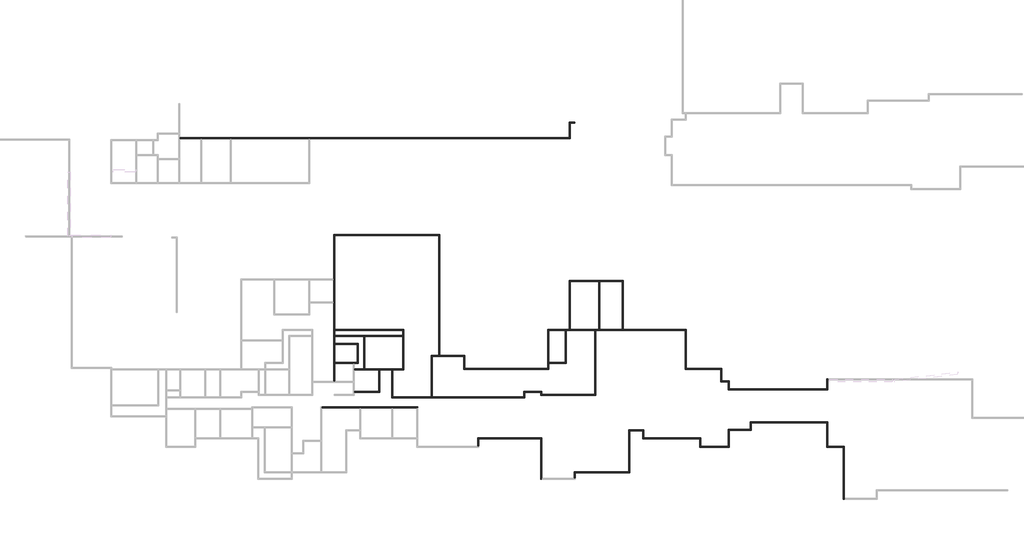
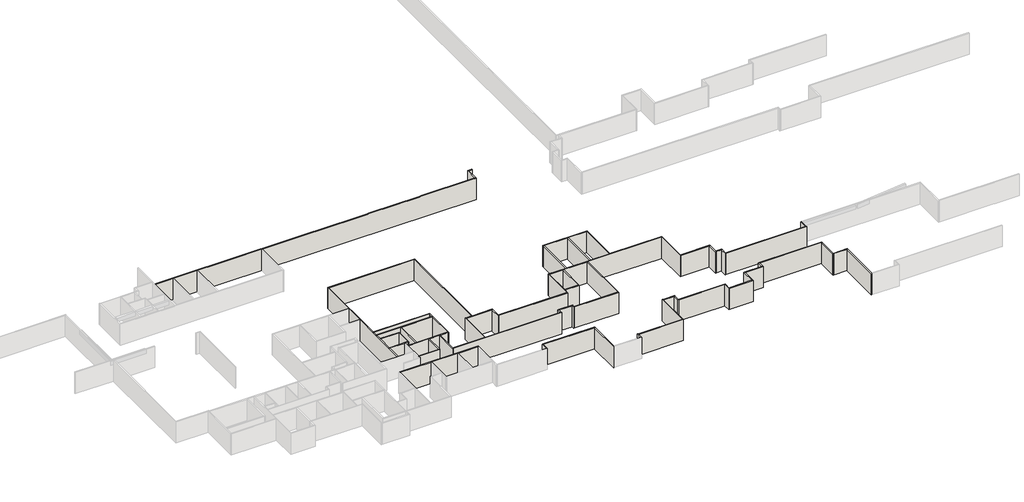
# One storey, part 3 of 8: 61 walls.
"""IFC4 building model written with IfcOpenShell, lengths in millimetres."""

import ifcopenshell
import ifcopenshell.guid

model = None  # the IFC model being written
_history = None  # IfcOwnerHistory: only IFC2X3 demands one
_inside = {}  # id of a spatial element -> (the spatial element, [elements in it])
_under = {}  # id of a project, library or spatial element -> (it, [spatial elements below it])
_declared = {}  # id of a project -> (the project, [libraries it declares])
_typed = {}  # id of a type object -> (the type object, [elements of that type])
_made_of = {}  # id of a material, layer set ... -> (it, [elements and type objects made of it])


def new_model(schema):
    """Start an empty IFC model of exactly this schema.

    Asked for "IFC4X3", IfcOpenShell would pick the latest addendum, in which some entities
    have other attributes; the version numbers below select the first issue.
    IFC2X3 requires an IfcOwnerHistory on every rooted entity: one is made here for all.
    """
    global model, _history
    if schema == "IFC4X3":
        model = ifcopenshell.file(schema_version=(4, 3, 0, 0))
    else:
        model = ifcopenshell.file(schema=schema)
    _inside.clear()
    _under.clear()
    _declared.clear()
    _typed.clear()
    _made_of.clear()
    _history = None
    if model.schema == "IFC2X3":
        org = make("IfcOrganization", Name="unknown")
        user = make(
            "IfcPersonAndOrganization",
            ThePerson=make("IfcPerson", FamilyName="unknown"),
            TheOrganization=org,
        )
        app = make(
            "IfcApplication",
            ApplicationDeveloper=org,
            Version="unknown",
            ApplicationFullName="unknown",
            ApplicationIdentifier="unknown",
        )
        _history = make(
            "IfcOwnerHistory",
            OwningUser=user,
            OwningApplication=app,
            ChangeAction="ADDED",
            CreationDate=0,
        )
    return model


def make(cls, **values):
    """One entity of the class cls with the attributes given. An attribute that is None is left unset."""
    return model.create_entity(
        cls, **{name: value for name, value in values.items() if value is not None}
    )


def rooted(cls, **values):
    """An entity with a GlobalId (a new one), such as an element, a storey or a relation."""
    return make(cls, GlobalId=ifcopenshell.guid.new(), OwnerHistory=_history, **values)


def si_unit(unit_type, name, prefix=None):
    """IfcSIUnit, for example si_unit("LENGTHUNIT", "METRE", prefix="MILLI")."""
    return make("IfcSIUnit", UnitType=unit_type, Prefix=prefix, Name=name)


def assignment(units):
    """IfcUnitAssignment: the units of a project."""
    return None if units is None else make("IfcUnitAssignment", Units=units)


def point(xyz):
    """IfcCartesianPoint."""
    return None if xyz is None else make("IfcCartesianPoint", Coordinates=xyz)


def direction(xyz):
    """IfcDirection."""
    return None if xyz is None else make("IfcDirection", DirectionRatios=xyz)


def frame(location, z_axis=None, x_axis=None):
    """IfcAxis2Placement3D, a coordinate frame: its origin and axes. An axis left out is left unset."""
    return make(
        "IfcAxis2Placement3D",
        Location=point(location),
        Axis=direction(z_axis),
        RefDirection=direction(x_axis),
    )


def origin():
    """The frame at (0, 0, 0) with its axes left unset."""
    return frame((0.0, 0.0, 0.0))


def origin_with_axes():
    """The frame at (0, 0, 0) with the z axis (0, 0, 1) and the x axis (1, 0, 0) written out."""
    return frame((0.0, 0.0, 0.0), z_axis=(0.0, 0.0, 1.0), x_axis=(1.0, 0.0, 0.0))


def place(relative_to, where):
    """IfcLocalPlacement: puts the frame where relative to a parent placement (None: the world)."""
    return make(
        "IfcLocalPlacement", PlacementRelTo=relative_to, RelativePlacement=where
    )


def context(
    kind, dimensions, precision=None, world=None, true_north=None, identifier=None
):
    """IfcGeometricRepresentationContext, for example the 3D "Model" context."""
    return make(
        "IfcGeometricRepresentationContext",
        ContextIdentifier=identifier,
        ContextType=kind,
        CoordinateSpaceDimension=dimensions,
        Precision=precision,
        WorldCoordinateSystem=world,
        TrueNorth=true_north,
    )


def project(units=None, contexts=None):
    """IfcProject with its units and contexts."""
    return rooted(
        "IfcProject",
        Name="project",
        RepresentationContexts=contexts,
        UnitsInContext=assignment(units),
    )


def spatial(cls, under=None, at=None, **own):
    """A site, building, storey or space (cls), placed at a placement, below another one or the project."""
    s = rooted(cls, ObjectPlacement=at, **own)
    if under is not None:
        _under.setdefault(under.id(), (under, []))[1].append(s)
    return s


def polyline(points):
    """IfcPolyline through the points."""
    return make("IfcPolyline", Points=[point(p) for p in points])


def outline(outer, holes=None, kind="AREA"):
    """IfcArbitraryClosedProfileDef: a profile drawn as a closed curve; with holes, ...WithVoids."""
    if holes is None:
        return make("IfcArbitraryClosedProfileDef", ProfileType=kind, OuterCurve=outer)
    return make(
        "IfcArbitraryProfileDefWithVoids",
        ProfileType=kind,
        OuterCurve=outer,
        InnerCurves=holes,
    )


def extrude(swept, where, along, depth):
    """IfcExtrudedAreaSolid: the profile swept, set in the frame where, extruded along a direction by depth."""
    return make(
        "IfcExtrudedAreaSolid",
        SweptArea=swept,
        Position=where,
        ExtrudedDirection=direction(along),
        Depth=depth,
    )


def faces_of(points, faces, orient=None, outer=None):
    """IfcFace entities. A face is a list of loops; a loop is a list of indices into points, from 0.

    orient and outer hold one flag for each loop. By default every Orientation is true, the
    first loop of a face is its IfcFaceOuterBound and the others are IfcFaceBound.
    """
    made = []
    for i, loops in enumerate(faces):
        bounds = []
        for j, loop in enumerate(loops):
            is_outer = j == 0 if outer is None else outer[i][j]
            bounds.append(
                make(
                    "IfcFaceOuterBound" if is_outer else "IfcFaceBound",
                    Bound=make("IfcPolyLoop", Polygon=[points[k] for k in loop]),
                    Orientation=True if orient is None else orient[i][j],
                )
            )
        made.append(make("IfcFace", Bounds=bounds))
    return made


def faceted_brep(points, faces, orient=None, outer=None, voids=None):
    """IfcFacetedBrep: a solid bounded by flat faces; with voids (closed shells), ...WithVoids."""
    shared = [point(p) for p in points]
    hull = make("IfcClosedShell", CfsFaces=faces_of(shared, faces, orient, outer))
    if voids is None:
        return make("IfcFacetedBrep", Outer=hull)
    return make(
        "IfcFacetedBrepWithVoids",
        Outer=hull,
        Voids=[
            make(cls, CfsFaces=faces_of(shared, fs, o, b)) for cls, fs, o, b in voids
        ],
    )


def shape(context_of_items, identifier, shape_type, items):
    """IfcShapeRepresentation: the items that make up one representation, for example the "Body"."""
    return make(
        "IfcShapeRepresentation",
        ContextOfItems=context_of_items,
        RepresentationIdentifier=identifier,
        RepresentationType=shape_type,
        Items=items,
    )


def made_of(thing, what):
    """Note that an element or type object is made of a material, layer set ...; save() writes the relation."""
    if what is not None:
        _made_of.setdefault(what.id(), (what, []))[1].append(thing)
    return thing


def element(
    cls,
    number,
    at=None,
    inside=None,
    cuts=None,
    type_object=None,
    material=None,
    context=None,
    identifier="Body",
    shape_type=None,
    held_by="IfcProductDefinitionShape",
    body=None,
    shapes=None,
    **own,
):
    """One element of the class cls, such as IfcWall. Its Tag is "e" and its number.

    at: its placement. inside: the storey or other place that contains it. cuts: it is an
    opening in that element (IfcRelVoidsElement). A single representation is given by context,
    identifier, shape_type and body (its items); several are given by shapes. held_by: the class
    of the entity that holds the representations. save() writes the other relations.
    """
    e = rooted(cls, Tag="e%d" % number, ObjectPlacement=at, **own)
    if body is not None:
        shapes = [shape(context, identifier, shape_type, body)]
    if shapes is not None:
        e.Representation = make(held_by, Representations=shapes)
    if inside is not None:
        _inside.setdefault(inside.id(), (inside, []))[1].append(e)
    if cuts is not None:
        rooted(
            "IfcRelVoidsElement", RelatingBuildingElement=cuts, RelatedOpeningElement=e
        )
    if type_object is not None:
        _typed.setdefault(type_object.id(), (type_object, []))[1].append(e)
    return made_of(e, material)


def aggregate(whole, parts):
    """IfcRelAggregates: a whole, such as a stair, and the parts it consists of."""
    return rooted("IfcRelAggregates", RelatingObject=whole, RelatedObjects=parts)


def save(model, path):
    """Write the relations noted so far, then the file.

    IfcRelAggregates (storeys below a building ...), IfcRelContainedInSpatialStructure (elements
    in a storey), IfcRelDefinesByType, IfcRelAssociatesMaterial and IfcRelDeclares: one each for
    every whole, place, type object, material and project.
    """
    for whole, parts in _under.values():
        aggregate(whole, parts)
    for where, things in _inside.values():
        rooted(
            "IfcRelContainedInSpatialStructure",
            RelatedElements=things,
            RelatingStructure=where,
        )
    for kind, things in _typed.values():
        rooted("IfcRelDefinesByType", RelatedObjects=things, RelatingType=kind)
    for what, things in _made_of.values():
        rooted("IfcRelAssociatesMaterial", RelatedObjects=things, RelatingMaterial=what)
    for by, libraries in _declared.values():
        rooted("IfcRelDeclares", RelatingContext=by, RelatedDefinitions=libraries)
    model.write(path)


model = new_model("IFC4")

# Units and contexts
model_context = context("Model", 3, world=origin())
ifc_project = project(units=[si_unit("LENGTHUNIT", "METRE", prefix="MILLI")], contexts=[model_context])

# Site, building, storey
site = spatial("IfcSite", under=ifc_project)
building = spatial("IfcBuilding", under=site)
storey = spatial("IfcBuildingStorey", under=building, Name="户型图", Elevation=0.0)

# Walls
placement = place(None, origin())
element("IfcWall", 1, ObjectType="所有墙体", at=placement, inside=storey, context=model_context, shape_type="Brep", body=[
    faceted_brep([(146227.9809999, 19565.6854079, 0.0), (146227.9809999, 20445.6854108, 0.0), (146227.9809999, 20565.6854108, 0.0), (146227.9809999, 20565.6854108, 3300.0), (146227.9809999, 20445.6854108, 3300.0), (146227.9809999, 19565.6854079, 3300.0), (146107.9809999, 19565.6854079, 0.0), (146107.9809999, 19565.6854079, 3300.0), (146107.9809999, 20565.6854108, 3300.0), (146107.9809999, 20565.6854108, 0.0)], [[[0, 1, 2, 3, 4, 5]], [[6, 7, 8, 9]], [[2, 1, 0, 6, 9]], [[5, 4, 3, 8, 7]], [[0, 5, 7, 6]], [[3, 2, 9, 8]]]),
])
element("IfcWall", 2, ObjectType="所有墙体", at=placement, inside=storey, context=model_context, shape_type="Brep", body=[
    faceted_brep([(146227.9809999, 20445.6854108, 0.0), (153757.9809859, 20445.6854108, 0.0), (153877.9809859, 20445.6854108, 0.0), (153877.9809859, 20445.6854108, 3300.0), (153757.9809859, 20445.6854108, 3300.0), (146227.9809999, 20445.6854108, 3300.0), (146227.9809999, 20565.6854108, 0.0), (146227.9809999, 20565.6854108, 3300.0), (153877.9809859, 20565.6854108, 3300.0), (153877.9809859, 20565.6854108, 0.0)], [[[0, 1, 2, 3, 4, 5]], [[6, 7, 8, 9]], [[2, 1, 0, 6, 9]], [[5, 4, 3, 8, 7]], [[0, 5, 7, 6]], [[3, 2, 9, 8]]]),
])
element("IfcWall", 3, ObjectType="所有墙体", at=placement, inside=storey, context=model_context, shape_type="Brep", body=[
    faceted_brep([(153757.9809859, 20445.6854108, 0.0), (153757.9809859, 15545.6854108, 0.0), (153757.9809859, 15545.6854108, 3300.0), (153757.9809859, 20445.6854108, 3300.0), (153877.9809859, 20445.6854108, 0.0), (153877.9809859, 20445.6854108, 3300.0), (153877.9809859, 15665.6854108, 3300.0), (153877.9809859, 15545.6854108, 3300.0), (153877.9809859, 15545.6854108, 0.0), (153877.9809859, 15665.6854108, 0.0)], [[[0, 1, 2, 3]], [[4, 5, 6, 7, 8, 9]], [[1, 0, 4, 9, 8]], [[3, 2, 7, 6, 5]], [[0, 3, 5, 4]], [[2, 1, 8, 7]]]),
])
element("IfcWall", 4, ObjectType="所有墙体", at=placement, inside=storey, context=model_context, shape_type="Brep", body=[
    faceted_brep([(157927.981003, 15665.6854108, 0.0), (157927.981003, 16345.6854097, 0.0), (157927.981003, 16465.6854097, 0.0), (157927.981003, 16465.6854097, 3300.0), (157927.981003, 16345.6854097, 3300.0), (157927.981003, 15665.6854108, 3300.0), (157807.981003, 15665.6854108, 0.0), (157807.981003, 15665.6854108, 3300.0), (157807.981003, 16465.6854097, 3300.0), (157807.981003, 16465.6854097, 0.0)], [[[0, 1, 2, 3, 4, 5]], [[6, 7, 8, 9]], [[2, 1, 0, 6, 9]], [[5, 4, 3, 8, 7]], [[0, 5, 7, 6]], [[3, 2, 9, 8]]]),
])
element("IfcWall", 5, ObjectType="所有墙体", at=placement, inside=storey, context=model_context, shape_type="Brep", body=[
    faceted_brep([(157927.981003, 16345.6854097, 0.0), (164527.9809935, 16345.6854097, 0.0), (164527.9809935, 16345.6854097, 3300.0), (157927.981003, 16345.6854097, 3300.0), (157927.981003, 16465.6854097, 0.0), (157927.981003, 16465.6854097, 3300.0), (164407.9809935, 16465.6854097, 3300.0), (164527.9809935, 16465.6854097, 3300.0), (164527.9809935, 16465.6854097, 0.0), (164407.9809935, 16465.6854097, 0.0)], [[[0, 1, 2, 3]], [[4, 5, 6, 7, 8, 9]], [[1, 0, 4, 9, 8]], [[3, 2, 7, 6, 5]], [[0, 3, 5, 4]], [[2, 1, 8, 7]]]),
])
element("IfcWall", 6, ObjectType="所有墙体", at=placement, inside=storey, context=model_context, shape_type="Brep", body=[
    faceted_brep([(164527.9809935, 16465.6854097, 0.0), (164527.9809935, 21420.9349261, 0.0), (164527.9809935, 21540.9349261, 0.0), (164527.9809935, 21540.9349261, 3300.0), (164527.9809935, 21420.9349261, 3300.0), (164527.9809935, 16465.6854097, 3300.0), (164407.9809935, 16465.6854097, 0.0), (164407.9809935, 16465.6854097, 3300.0), (164407.9809935, 21540.9349261, 3300.0), (164407.9809935, 21540.9349261, 0.0)], [[[0, 1, 2, 3, 4, 5]], [[6, 7, 8, 9]], [[2, 1, 0, 6, 9]], [[5, 4, 3, 8, 7]], [[0, 5, 7, 6]], [[3, 2, 9, 8]]]),
])
element("IfcWall", 7, ObjectType="所有墙体", at=placement, inside=storey, context=model_context, shape_type="Brep", body=[
    faceted_brep([(164527.9809935, 21420.9349261, 0.0), (166107.9809965, 21420.9349261, 0.0), (166227.9809965, 21420.9349261, 0.0), (166227.9809965, 21420.9349261, 3300.0), (166107.9809965, 21420.9349261, 3300.0), (164527.9809935, 21420.9349261, 3300.0), (164527.9809935, 21540.9349261, 0.0), (164527.9809935, 21540.9349261, 3300.0), (166227.9809965, 21540.9349261, 3300.0), (166227.9809965, 21540.9349261, 0.0)], [[[0, 1, 2, 3, 4, 5]], [[6, 7, 8, 9]], [[2, 1, 0, 6, 9]], [[5, 4, 3, 8, 7]], [[0, 5, 7, 6]], [[3, 2, 9, 8]]]),
])
element("IfcWall", 8, ObjectType="所有墙体", at=placement, inside=storey, context=model_context, shape_type="Brep", body=[
    faceted_brep([(166107.9809965, 21420.9349261, 0.0), (166107.9809965, 20445.6854108, 0.0), (166107.9809965, 20445.6854108, 3300.0), (166107.9809965, 21420.9349261, 3300.0), (166227.9809965, 21420.9349261, 0.0), (166227.9809965, 21420.9349261, 3300.0), (166227.9809965, 20565.6854108, 3300.0), (166227.9809965, 20445.6854108, 3300.0), (166227.9809965, 20445.6854108, 0.0), (166227.9809965, 20565.6854108, 0.0)], [[[0, 1, 2, 3]], [[4, 5, 6, 7, 8, 9]], [[1, 0, 4, 9, 8]], [[3, 2, 7, 6, 5]], [[0, 3, 5, 4]], [[2, 1, 8, 7]]]),
])
element("IfcWall", 9, ObjectType="所有墙体", at=placement, inside=storey, context=model_context, shape_type="Brep", body=[
    faceted_brep([(166227.9809965, 20445.6854108, 0.0), (173007.9809872, 20445.6854108, 0.0), (173127.9809872, 20445.6854108, 0.0), (173127.9809872, 20445.6854108, 3300.0), (173007.9809872, 20445.6854108, 3300.0), (166227.9809965, 20445.6854108, 3300.0), (166227.9809965, 20565.6854108, 0.0), (166227.9809965, 20565.6854108, 3300.0), (173127.9809872, 20565.6854108, 3300.0), (173127.9809872, 20565.6854108, 0.0)], [[[0, 1, 2, 3, 4, 5]], [[6, 7, 8, 9]], [[2, 1, 0, 6, 9]], [[5, 4, 3, 8, 7]], [[0, 5, 7, 6]], [[3, 2, 9, 8]]]),
])
element("IfcWall", 10, ObjectType="所有墙体", at=placement, inside=storey, context=model_context, shape_type="Brep", body=[
    faceted_brep([(173007.9809872, 20445.6854108, 0.0), (173007.9809872, 19445.6854134, 0.0), (173007.9809872, 19445.6854134, 3300.0), (173007.9809872, 20445.6854108, 3300.0), (173127.9809872, 20445.6854108, 0.0), (173127.9809872, 20445.6854108, 3300.0), (173127.9809872, 19565.6854134, 3300.0), (173127.9809872, 19445.6854134, 3300.0), (173127.9809872, 19445.6854134, 0.0), (173127.9809872, 19565.6854134, 0.0)], [[[0, 1, 2, 3]], [[4, 5, 6, 7, 8, 9]], [[1, 0, 4, 9, 8]], [[3, 2, 7, 6, 5]], [[0, 3, 5, 4]], [[2, 1, 8, 7]]]),
])
element("IfcWall", 11, ObjectType="所有墙体", at=placement, inside=storey, context=model_context, shape_type="Brep", body=[
    faceted_brep([(173127.9809872, 19445.6854134, 0.0), (176627.9809932, 19445.6854134, 0.0), (176627.9809932, 19445.6854134, 3300.0), (173127.9809872, 19445.6854134, 3300.0), (173127.9809872, 19565.6854134, 0.0), (173127.9809872, 19565.6854134, 3300.0), (176507.9809932, 19565.6854134, 3300.0), (176627.9809932, 19565.6854134, 3300.0), (176627.9809932, 19565.6854134, 0.0), (176507.9809932, 19565.6854134, 0.0)], [[[0, 1, 2, 3]], [[4, 5, 6, 7, 8, 9]], [[1, 0, 4, 9, 8]], [[3, 2, 7, 6, 5]], [[0, 3, 5, 4]], [[2, 1, 8, 7]]]),
])
element("IfcWall", 12, ObjectType="所有墙体", at=placement, inside=storey, context=model_context, shape_type="Brep", body=[
    faceted_brep([(176627.9809932, 19565.6854134, 0.0), (176627.9809932, 21496.1844416, 0.0), (176627.9809932, 21616.1844416, 0.0), (176627.9809932, 21616.1844416, 3300.0), (176627.9809932, 21496.1844416, 3300.0), (176627.9809932, 19565.6854134, 3300.0), (176507.9809932, 19565.6854134, 0.0), (176507.9809932, 19565.6854134, 3300.0), (176507.9809932, 21616.1844416, 3300.0), (176507.9809932, 21616.1844416, 0.0)], [[[0, 1, 2, 3, 4, 5]], [[6, 7, 8, 9]], [[2, 1, 0, 6, 9]], [[5, 4, 3, 8, 7]], [[0, 5, 7, 6]], [[3, 2, 9, 8]]]),
])
element("IfcWall", 13, ObjectType="所有墙体", at=placement, inside=storey, context=model_context, shape_type="Brep", body=[
    faceted_brep([(176627.9809932, 21496.1844416, 0.0), (179277.9850002, 21496.1844416, 0.0), (179277.9850002, 21496.1844416, 3300.0), (176627.9809932, 21496.1844416, 3300.0), (176627.9809932, 21616.1844416, 0.0), (176627.9809932, 21616.1844416, 3300.0), (179157.9850002, 21616.1844416, 3300.0), (179277.9850002, 21616.1844416, 3300.0), (179277.9850002, 21616.1844416, 0.0), (179157.9850002, 21616.1844416, 0.0)], [[[0, 1, 2, 3]], [[4, 5, 6, 7, 8, 9]], [[1, 0, 4, 9, 8]], [[3, 2, 7, 6, 5]], [[0, 3, 5, 4]], [[2, 1, 8, 7]]]),
])
element("IfcWall", 14, ObjectType="所有墙体", at=placement, inside=storey, context=model_context, shape_type="Brep", body=[
    faceted_brep([(179277.9850002, 21616.1844416, 0.0), (179277.9850002, 22396.1673448, 0.0), (179277.9850002, 22516.1673448, 0.0), (179277.9850002, 22516.1673448, 3300.0), (179277.9850002, 22396.1673448, 3300.0), (179277.9850002, 21616.1844416, 3300.0), (179157.9850002, 21616.1844416, 0.0), (179157.9850002, 21616.1844416, 3300.0), (179157.9850002, 22516.1673448, 3300.0), (179157.9850002, 22516.1673448, 0.0)], [[[0, 1, 2, 3, 4, 5]], [[6, 7, 8, 9]], [[2, 1, 0, 6, 9]], [[5, 4, 3, 8, 7]], [[0, 5, 7, 6]], [[3, 2, 9, 8]]]),
])
element("IfcWall", 15, ObjectType="所有墙体", at=placement, inside=storey, context=model_context, shape_type="Brep", body=[
    faceted_brep([(179277.9850002, 22396.1673448, 0.0), (188413.8473665, 22396.1673448, 0.0), (188533.8473665, 22396.1673448, 0.0), (188533.8473665, 22396.1673448, 3300.0), (188413.8473665, 22396.1673448, 3300.0), (179277.9850002, 22396.1673448, 3300.0), (179277.9850002, 22516.1673448, 0.0), (179277.9850002, 22516.1673448, 3300.0), (188533.8473665, 22516.1673448, 3300.0), (188533.8473665, 22516.1673448, 0.0)], [[[0, 1, 2, 3, 4, 5]], [[6, 7, 8, 9]], [[2, 1, 0, 6, 9]], [[5, 4, 3, 8, 7]], [[0, 5, 7, 6]], [[3, 2, 9, 8]]]),
])
element("IfcWall", 16, ObjectType="所有墙体", at=placement, inside=storey, context=model_context, shape_type="Brep", body=[
    faceted_brep([(188413.8473665, 22396.1673448, 0.0), (188413.8473665, 19445.6854134, 0.0), (188413.8473665, 19445.6854134, 3300.0), (188413.8473665, 22396.1673448, 3300.0), (188533.8473665, 22396.1673448, 0.0), (188533.8473665, 22396.1673448, 3300.0), (188533.8473665, 19565.6854134, 3300.0), (188533.8473665, 19445.6854134, 3300.0), (188533.8473665, 19445.6854134, 0.0), (188533.8473665, 19565.6854134, 0.0)], [[[0, 1, 2, 3]], [[4, 5, 6, 7, 8, 9]], [[1, 0, 4, 9, 8]], [[3, 2, 7, 6, 5]], [[0, 3, 5, 4]], [[2, 1, 8, 7]]]),
])
element("IfcWall", 17, ObjectType="所有墙体", at=placement, inside=storey, context=model_context, shape_type="Brep", body=[
    faceted_brep([(188533.8473665, 19445.6854134, 0.0), (190464.1761986, 19445.6854134, 0.0), (190584.1761986, 19445.6854134, 0.0), (190584.1761986, 19445.6854134, 3300.0), (190464.1761986, 19445.6854134, 3300.0), (188533.8473665, 19445.6854134, 3300.0), (188533.8473665, 19565.6854134, 0.0), (188533.8473665, 19565.6854134, 3300.0), (190584.1761986, 19565.6854134, 3300.0), (190584.1761986, 19565.6854134, 0.0)], [[[0, 1, 2, 3, 4, 5]], [[6, 7, 8, 9]], [[2, 1, 0, 6, 9]], [[5, 4, 3, 8, 7]], [[0, 5, 7, 6]], [[3, 2, 9, 8]]]),
])
element("IfcWall", 18, ObjectType="所有墙体", at=placement, inside=storey, context=model_context, shape_type="Brep", body=[
    faceted_brep([(190464.1761986, 19445.6854134, 0.0), (190464.1761986, 13145.7645172, 0.0), (190464.1761986, 13145.7645172, 3300.0), (190464.1761986, 19445.6854134, 3300.0), (190584.1761986, 19445.6854134, 0.0), (190584.1761986, 19445.6854134, 3300.0), (190584.1761986, 13265.7645172, 3300.0), (190584.1761986, 13145.7645172, 3300.0), (190584.1761986, 13145.7645172, 0.0), (190584.1761986, 13265.7645172, 0.0)], [[[0, 1, 2, 3]], [[4, 5, 6, 7, 8, 9]], [[1, 0, 4, 9, 8]], [[3, 2, 7, 6, 5]], [[0, 3, 5, 4]], [[2, 1, 8, 7]]]),
])
element("IfcWall", 19, ObjectType="所有墙体", at=placement, inside=storey, context=model_context, shape_type="Brep", body=[
    faceted_brep([(128682.9654795, 45156.8473862, 0.0), (128802.9654795, 45156.8473862, 0.0), (141413.8359011, 45156.8473862, 0.0), (141533.8359011, 45156.8473862, 0.0), (141533.8359011, 45156.8473862, 3300.0), (141413.8359011, 45156.8473862, 3300.0), (128802.9654795, 45156.8473862, 3300.0), (128682.9654795, 45156.8473862, 3300.0), (128682.9654795, 45276.8473862, 0.0), (128682.9654795, 45276.8473862, 3300.0), (141533.8359011, 45276.8473862, 3300.0), (141533.8359011, 45276.8473862, 0.0)], [[[0, 1, 2, 3, 4, 5, 6, 7]], [[8, 9, 10, 11]], [[3, 2, 1, 0, 8, 11]], [[7, 6, 5, 4, 10, 9]], [[4, 3, 11, 10]], [[0, 7, 9, 8]]]),
])
element("IfcWall", 20, ObjectType="所有墙体", at=placement, inside=storey, context=model_context, shape_type="SweptSolid", body=[
    extrude(outline(polyline([(141413.8359011, 30576.8473862), (141413.8359011, 45156.8473862), (141533.8359011, 45156.8473862), (141533.8359011, 30576.8473862), (141413.8359011, 30576.8473862)])), origin_with_axes(), (0.0, 0.0, 1.0), 3300.0),
])
element("IfcWall", 21, ObjectType="所有墙体", at=placement, inside=storey, context=model_context, shape_type="Brep", body=[
    faceted_brep([(140627.9809914, 30456.8473862, 0.0), (144408.4809802, 30456.8473862, 0.0), (144528.4809802, 30456.8473862, 0.0), (144528.4809802, 30456.8473862, 3300.0), (144408.4809802, 30456.8473862, 3300.0), (140627.9809914, 30456.8473862, 3300.0), (140627.9809914, 30576.8473862, 0.0), (140627.9809914, 30576.8473862, 3300.0), (141413.8359011, 30576.8473862, 3300.0), (141533.8359011, 30576.8473862, 3300.0), (144528.4809802, 30576.8473862, 3300.0), (144528.4809802, 30576.8473862, 0.0), (141533.8359011, 30576.8473862, 0.0), (141413.8359011, 30576.8473862, 0.0)], [[[0, 1, 2, 3, 4, 5]], [[6, 7, 8, 9, 10, 11, 12, 13]], [[2, 1, 0, 6, 13, 12, 11]], [[5, 4, 3, 10, 9, 8, 7]], [[3, 2, 11, 10]], [[0, 5, 7, 6]]]),
])
element("IfcWall", 22, ObjectType="所有墙体", at=placement, inside=storey, context=model_context, shape_type="Brep", body=[
    faceted_brep([(144408.4809802, 30456.8473862, 0.0), (144408.4809802, 28910.6856669, 0.0), (144408.4809802, 28910.6856669, 3300.0), (144408.4809802, 30456.8473862, 3300.0), (144528.4809802, 30456.8473862, 0.0), (144528.4809802, 30456.8473862, 3300.0), (144528.4809802, 29030.6856669, 3300.0), (144528.4809802, 28910.6856669, 3300.0), (144528.4809802, 28910.6856669, 0.0), (144528.4809802, 29030.6856669, 0.0)], [[[0, 1, 2, 3]], [[4, 5, 6, 7, 8, 9]], [[1, 0, 4, 9, 8]], [[3, 2, 7, 6, 5]], [[0, 3, 5, 4]], [[2, 1, 8, 7]]]),
])
element("IfcWall", 23, ObjectType="所有墙体", at=placement, inside=storey, context=model_context, shape_type="Brep", body=[
    faceted_brep([(144528.4809802, 28910.6856669, 0.0), (154728.4809802, 28910.6856669, 0.0), (154728.4809802, 28910.6856669, 3300.0), (144528.4809802, 28910.6856669, 3300.0), (144528.4809802, 29030.6856669, 0.0), (144528.4809802, 29030.6856669, 3300.0), (154608.4809802, 29030.6856669, 3300.0), (154728.4809802, 29030.6856669, 3300.0), (154728.4809802, 29030.6856669, 0.0), (154608.4809802, 29030.6856669, 0.0)], [[[0, 1, 2, 3]], [[4, 5, 6, 7, 8, 9]], [[1, 0, 4, 9, 8]], [[3, 2, 7, 6, 5]], [[0, 3, 5, 4]], [[2, 1, 8, 7]]]),
])
element("IfcWall", 24, ObjectType="所有墙体", at=placement, inside=storey, context=model_context, shape_type="Brep", body=[
    faceted_brep([(154728.4809802, 29030.6856669, 0.0), (154728.4809802, 29595.6854131, 0.0), (154728.4809802, 29715.6854131, 0.0), (154728.4809802, 33645.6854155, 0.0), (154728.4809802, 33645.6854155, 3300.0), (154728.4809802, 29715.6854131, 3300.0), (154728.4809802, 29595.6854131, 3300.0), (154728.4809802, 29030.6856669, 3300.0), (154608.4809802, 29030.6856669, 0.0), (154608.4809802, 29030.6856669, 3300.0), (154608.4809802, 33645.6854155, 3300.0), (154608.4809802, 33645.6854155, 0.0)], [[[0, 1, 2, 3, 4, 5, 6, 7]], [[8, 9, 10, 11]], [[3, 2, 1, 0, 8, 11]], [[7, 6, 5, 4, 10, 9]], [[0, 7, 9, 8]], [[4, 3, 11, 10]]]),
])
element("IfcWall", 25, ObjectType="所有墙体", at=placement, inside=storey, context=model_context, shape_type="Brep", body=[
    faceted_brep([(154728.4809802, 29595.6854131, 0.0), (156827.9809916, 29595.6854131, 0.0), (156827.9809916, 29595.6854131, 3300.0), (154728.4809802, 29595.6854131, 3300.0), (154728.4809802, 29715.6854131, 0.0), (154728.4809802, 29715.6854131, 3300.0), (156707.9809916, 29715.6854131, 3300.0), (156827.9809916, 29715.6854131, 3300.0), (156827.9809916, 29715.6854131, 0.0), (156707.9809916, 29715.6854131, 0.0)], [[[0, 1, 2, 3]], [[4, 5, 6, 7, 8, 9]], [[1, 0, 4, 9, 8]], [[3, 2, 7, 6, 5]], [[0, 3, 5, 4]], [[2, 1, 8, 7]]]),
])
element("IfcWall", 26, ObjectType="所有墙体", at=placement, inside=storey, context=model_context, shape_type="SweptSolid", body=[
    extrude(outline(polyline([(156827.9809916, 33645.6854155), (156827.9809916, 29715.6854131), (156707.9809916, 29715.6854131), (156707.9809916, 33645.6854155), (156827.9809916, 33645.6854155)])), origin_with_axes(), (0.0, 0.0, 1.0), 3300.0),
])
element("IfcWall", 27, ObjectType="所有墙体", at=placement, inside=storey, context=model_context, shape_type="Brep", body=[
    faceted_brep([(171427.9810052, 33765.6854155, 0.0), (163752.9781417, 33765.6854155, 0.0), (163632.9781417, 33765.6854155, 0.0), (160903.0268476, 33765.6854155, 0.0), (160783.0268476, 33765.6854155, 0.0), (157358.8240567, 33765.6854155, 0.0), (157238.8240567, 33765.6854155, 0.0), (154608.4809802, 33765.6854155, 0.0), (154608.4809802, 33765.6854155, 3300.0), (157238.8240567, 33765.6854155, 3300.0), (157358.8240567, 33765.6854155, 3300.0), (160783.0268476, 33765.6854155, 3300.0), (160903.0268476, 33765.6854155, 3300.0), (163632.9781417, 33765.6854155, 3300.0), (163752.9781417, 33765.6854155, 3300.0), (171427.9810052, 33765.6854155, 3300.0), (171427.9810052, 33645.6854155, 0.0), (171427.9810052, 33645.6854155, 3300.0), (171307.9810052, 33645.6854155, 3300.0), (160427.9809891, 33645.6854155, 3300.0), (160307.9809891, 33645.6854155, 3300.0), (156827.9809916, 33645.6854155, 3300.0), (156707.9809916, 33645.6854155, 3300.0), (154728.4809802, 33645.6854155, 3300.0), (154608.4809802, 33645.6854155, 3300.0), (154608.4809802, 33645.6854155, 0.0), (154728.4809802, 33645.6854155, 0.0), (156707.9809916, 33645.6854155, 0.0), (156827.9809916, 33645.6854155, 0.0), (160307.9809891, 33645.6854155, 0.0), (160427.9809891, 33645.6854155, 0.0), (171307.9810052, 33645.6854155, 0.0)], [[[0, 1, 2, 3, 4, 5, 6, 7, 8, 9, 10, 11, 12, 13, 14, 15]], [[16, 17, 18, 19, 20, 21, 22, 23, 24, 25, 26, 27, 28, 29, 30, 31]], [[7, 6, 5, 4, 3, 2, 1, 0, 16, 31, 30, 29, 28, 27, 26, 25]], [[15, 14, 13, 12, 11, 10, 9, 8, 24, 23, 22, 21, 20, 19, 18, 17]], [[8, 7, 25, 24]], [[0, 15, 17, 16]]]),
])
element("IfcWall", 28, ObjectType="所有墙体", at=placement, inside=storey, context=model_context, shape_type="SweptSolid", body=[
    extrude(outline(polyline([(160903.0268476, 39545.6854155), (160903.0268476, 33765.6854155), (160783.0268476, 33765.6854155), (160783.0268476, 39545.6854155), (160903.0268476, 39545.6854155)])), origin_with_axes(), (0.0, 0.0, 1.0), 3300.0),
])
element("IfcWall", 29, ObjectType="所有墙体", at=placement, inside=storey, context=model_context, shape_type="Brep", body=[
    faceted_brep([(163752.9781417, 39665.6854155, 0.0), (157238.8240567, 39665.6854155, 0.0), (157238.8240567, 39665.6854155, 3300.0), (163752.9781417, 39665.6854155, 3300.0), (163752.9781417, 39545.6854155, 0.0), (163752.9781417, 39545.6854155, 3300.0), (163632.9781417, 39545.6854155, 3300.0), (160903.0268476, 39545.6854155, 3300.0), (160783.0268476, 39545.6854155, 3300.0), (157358.8240567, 39545.6854155, 3300.0), (157238.8240567, 39545.6854155, 3300.0), (157238.8240567, 39545.6854155, 0.0), (157358.8240567, 39545.6854155, 0.0), (160783.0268476, 39545.6854155, 0.0), (160903.0268476, 39545.6854155, 0.0), (163632.9781417, 39545.6854155, 0.0)], [[[0, 1, 2, 3]], [[4, 5, 6, 7, 8, 9, 10, 11, 12, 13, 14, 15]], [[1, 0, 4, 15, 14, 13, 12, 11]], [[3, 2, 10, 9, 8, 7, 6, 5]], [[2, 1, 11, 10]], [[0, 3, 5, 4]]]),
])
element("IfcWall", 30, ObjectType="所有墙体", at=placement, inside=storey, context=model_context, shape_type="SweptSolid", body=[
    extrude(outline(polyline([(157238.8240567, 33765.6854155), (157238.8240567, 39545.6854155), (157358.8240567, 39545.6854155), (157358.8240567, 33765.6854155), (157238.8240567, 33765.6854155)])), origin_with_axes(), (0.0, 0.0, 1.0), 3300.0),
])
element("IfcWall", 31, ObjectType="所有墙体", at=placement, inside=storey, context=model_context, shape_type="SweptSolid", body=[
    extrude(outline(polyline([(163632.9781417, 33765.6854155), (163632.9781417, 39545.6854155), (163752.9781417, 39545.6854155), (163752.9781417, 33765.6854155), (163632.9781417, 33765.6854155)])), origin_with_axes(), (0.0, 0.0, 1.0), 3300.0),
])
element("IfcWall", 32, ObjectType="所有墙体", at=placement, inside=storey, context=model_context, shape_type="Brep", body=[
    faceted_brep([(171307.9810052, 33645.6854155, 0.0), (171307.9810052, 28910.6856669, 0.0), (171307.9810052, 28910.6856669, 3300.0), (171307.9810052, 33645.6854155, 3300.0), (171427.9810052, 33645.6854155, 0.0), (171427.9810052, 33645.6854155, 3300.0), (171427.9810052, 29030.6856669, 3300.0), (171427.9810052, 28910.6856669, 3300.0), (171427.9810052, 28910.6856669, 0.0), (171427.9810052, 29030.6856669, 0.0)], [[[0, 1, 2, 3]], [[4, 5, 6, 7, 8, 9]], [[1, 0, 4, 9, 8]], [[3, 2, 7, 6, 5]], [[0, 3, 5, 4]], [[2, 1, 8, 7]]]),
])
element("IfcWall", 33, ObjectType="所有墙体", at=placement, inside=storey, context=model_context, shape_type="Brep", body=[
    faceted_brep([(171427.9810052, 28910.6856669, 0.0), (175607.9810895, 28910.6856669, 0.0), (175727.9810895, 28910.6856669, 0.0), (175727.9810895, 28910.6856669, 3300.0), (175607.9810895, 28910.6856669, 3300.0), (171427.9810052, 28910.6856669, 3300.0), (171427.9810052, 29030.6856669, 0.0), (171427.9810052, 29030.6856669, 3300.0), (175727.9810895, 29030.6856669, 3300.0), (175727.9810895, 29030.6856669, 0.0)], [[[0, 1, 2, 3, 4, 5]], [[6, 7, 8, 9]], [[2, 1, 0, 6, 9]], [[5, 4, 3, 8, 7]], [[0, 5, 7, 6]], [[3, 2, 9, 8]]]),
])
element("IfcWall", 34, ObjectType="所有墙体", at=placement, inside=storey, context=model_context, shape_type="Brep", body=[
    faceted_brep([(175607.9810895, 28910.6856669, 0.0), (175607.9810895, 27370.687934, 0.0), (175607.9810895, 27370.687934, 3300.0), (175607.9810895, 28910.6856669, 3300.0), (175727.9810895, 28910.6856669, 0.0), (175727.9810895, 28910.6856669, 3300.0), (175727.9810895, 27490.687934, 3300.0), (175727.9810895, 27370.687934, 3300.0), (175727.9810895, 27370.687934, 0.0), (175727.9810895, 27490.687934, 0.0)], [[[0, 1, 2, 3]], [[4, 5, 6, 7, 8, 9]], [[1, 0, 4, 9, 8]], [[3, 2, 7, 6, 5]], [[0, 3, 5, 4]], [[2, 1, 8, 7]]]),
])
element("IfcWall", 35, ObjectType="所有墙体", at=placement, inside=storey, context=model_context, shape_type="Brep", body=[
    faceted_brep([(175727.9810895, 27370.687934, 0.0), (176507.9809932, 27370.687934, 0.0), (176627.9809932, 27370.687934, 0.0), (176627.9809932, 27370.687934, 3300.0), (176507.9809932, 27370.687934, 3300.0), (175727.9810895, 27370.687934, 3300.0), (175727.9810895, 27490.687934, 0.0), (175727.9810895, 27490.687934, 3300.0), (176627.9809932, 27490.687934, 3300.0), (176627.9809932, 27490.687934, 0.0)], [[[0, 1, 2, 3, 4, 5]], [[6, 7, 8, 9]], [[2, 1, 0, 6, 9]], [[5, 4, 3, 8, 7]], [[0, 5, 7, 6]], [[3, 2, 9, 8]]]),
])
element("IfcWall", 36, ObjectType="所有墙体", at=placement, inside=storey, context=model_context, shape_type="Brep", body=[
    faceted_brep([(176507.9809932, 27370.687934, 0.0), (176507.9809932, 26395.6879034, 0.0), (176507.9809932, 26395.6879034, 3300.0), (176507.9809932, 27370.687934, 3300.0), (176627.9809932, 27370.687934, 0.0), (176627.9809932, 27370.687934, 3300.0), (176627.9809932, 26515.6879034, 3300.0), (176627.9809932, 26395.6879034, 3300.0), (176627.9809932, 26395.6879034, 0.0), (176627.9809932, 26515.6879034, 0.0)], [[[0, 1, 2, 3]], [[4, 5, 6, 7, 8, 9]], [[1, 0, 4, 9, 8]], [[3, 2, 7, 6, 5]], [[0, 3, 5, 4]], [[2, 1, 8, 7]]]),
])
element("IfcWall", 37, ObjectType="所有墙体", at=placement, inside=storey, context=model_context, shape_type="Brep", body=[
    faceted_brep([(176627.9809932, 26395.6879034, 0.0), (188533.8473665, 26395.6879034, 0.0), (188533.8473665, 26395.6879034, 3300.0), (176627.9809932, 26395.6879034, 3300.0), (176627.9809932, 26515.6879034, 0.0), (176627.9809932, 26515.6879034, 3300.0), (188413.8473665, 26515.6879034, 3300.0), (188533.8473665, 26515.6879034, 3300.0), (188533.8473665, 26515.6879034, 0.0), (188413.8473665, 26515.6879034, 0.0)], [[[0, 1, 2, 3]], [[4, 5, 6, 7, 8, 9]], [[1, 0, 4, 9, 8]], [[3, 2, 7, 6, 5]], [[0, 3, 5, 4]], [[2, 1, 8, 7]]]),
])
element("IfcWall", 38, ObjectType="所有墙体", at=placement, inside=storey, context=model_context, shape_type="Brep", body=[
    faceted_brep([(188533.8473665, 26515.6879034, 0.0), (188533.8473665, 27606.8378863, 0.0), (188533.8473665, 27726.8378863, 0.0), (188533.8473665, 27726.8378863, 3300.0), (188533.8473665, 27606.8378863, 3300.0), (188533.8473665, 26515.6879034, 3300.0), (188413.8473665, 26515.6879034, 0.0), (188413.8473665, 26515.6879034, 3300.0), (188413.8473665, 27726.8378863, 3300.0), (188413.8473665, 27726.8378863, 0.0)], [[[0, 1, 2, 3, 4, 5]], [[6, 7, 8, 9]], [[2, 1, 0, 6, 9]], [[5, 4, 3, 8, 7]], [[0, 5, 7, 6]], [[3, 2, 9, 8]]]),
])
element("IfcWall", 39, ObjectType="所有墙体", at=placement, inside=storey, context=model_context, shape_type="Brep", body=[
    faceted_brep([(128682.9654795, 45156.8473862, 0.0), (128682.9654795, 39876.8473862, 0.0), (128682.9654795, 39756.8473862, 0.0), (128682.9654795, 37051.6496402, 0.0), (128682.9654795, 36931.6496402, 0.0), (128682.9654795, 27451.6496402, 0.0), (128682.9654795, 27451.6496402, 3300.0), (128682.9654795, 36931.6496402, 3300.0), (128682.9654795, 37051.6496402, 3300.0), (128682.9654795, 39756.8473862, 3300.0), (128682.9654795, 39876.8473862, 3300.0), (128682.9654795, 45156.8473862, 3300.0), (128802.9654795, 45156.8473862, 0.0), (128802.9654795, 45156.8473862, 3300.0), (128802.9654795, 33765.6854157, 3300.0), (128802.9654795, 33645.6854157, 3300.0), (128802.9654795, 32990.685413, 3300.0), (128802.9654795, 32870.685413, 3300.0), (128802.9654795, 32040.6854089, 3300.0), (128802.9654795, 31920.6854089, 3300.0), (128802.9654795, 29715.6854131, 3300.0), (128802.9654795, 29595.6854131, 3300.0), (128802.9654795, 27451.6496402, 3300.0), (128802.9654795, 27451.6496402, 0.0), (128802.9654795, 29595.6854131, 0.0), (128802.9654795, 29715.6854131, 0.0), (128802.9654795, 31920.6854089, 0.0), (128802.9654795, 32040.6854089, 0.0), (128802.9654795, 32870.685413, 0.0), (128802.9654795, 32990.685413, 0.0), (128802.9654795, 33645.6854157, 0.0), (128802.9654795, 33765.6854157, 0.0)], [[[0, 1, 2, 3, 4, 5, 6, 7, 8, 9, 10, 11]], [[12, 13, 14, 15, 16, 17, 18, 19, 20, 21, 22, 23, 24, 25, 26, 27, 28, 29, 30, 31]], [[5, 4, 3, 2, 1, 0, 12, 31, 30, 29, 28, 27, 26, 25, 24, 23]], [[11, 10, 9, 8, 7, 6, 22, 21, 20, 19, 18, 17, 16, 15, 14, 13]], [[0, 11, 13, 12]], [[6, 5, 23, 22]]]),
])
element("IfcWall", 40, ObjectType="所有墙体", at=placement, inside=storey, context=model_context, shape_type="Brep", body=[
    faceted_brep([(109958.7128377, 56907.0370398, 0.0), (125638.8240412, 56907.0370398, 0.0), (125758.8240412, 56907.0370398, 0.0), (157358.8240567, 56907.0370398, 0.0), (157358.8240567, 56907.0370398, 3300.0), (157226.4248507, 56907.0370398, 3300.0), (156926.4248507, 56907.0370398, 3300.0), (149326.4248507, 56907.0370398, 3300.0), (149026.4248507, 56907.0370398, 3300.0), (141526.4248507, 56907.0370398, 3300.0), (141226.4248507, 56907.0370398, 3300.0), (133626.4248507, 56907.0370398, 3300.0), (133326.4248507, 56907.0370398, 3300.0), (125848.8240412, 56907.0370398, 3300.0), (125758.8240412, 56907.0370398, 3300.0), (125638.8240412, 56907.0370398, 3300.0), (125548.8240412, 56907.0370398, 3300.0), (117798.8477351, 56907.0370398, 3300.0), (117498.8477351, 56907.0370398, 3300.0), (109958.7128377, 56907.0370398, 3300.0), (109958.7128377, 57027.0370398, 0.0), (109958.7128377, 57027.0370398, 3300.0), (117498.8477351, 57027.0370398, 3300.0), (117798.8477351, 57027.0370398, 3300.0), (125548.8240412, 57027.0370398, 3300.0), (125848.8240412, 57027.0370398, 3300.0), (133326.4248507, 57027.0370398, 3300.0), (133626.4248507, 57027.0370398, 3300.0), (141226.4248507, 57027.0370398, 3300.0), (141526.4248507, 57027.0370398, 3300.0), (149026.4248507, 57027.0370398, 3300.0), (149326.4248507, 57027.0370398, 3300.0), (156926.4248507, 57027.0370398, 3300.0), (157226.4248507, 57027.0370398, 3300.0), (157238.8240567, 57027.0370398, 3300.0), (157358.8240567, 57027.0370398, 3300.0), (157358.8240567, 57027.0370398, 0.0), (157238.8240567, 57027.0370398, 0.0)], [[[0, 1, 2, 3, 4, 5, 6, 7, 8, 9, 10, 11, 12, 13, 14, 15, 16, 17, 18, 19]], [[20, 21, 22, 23, 24, 25, 26, 27, 28, 29, 30, 31, 32, 33, 34, 35, 36, 37]], [[3, 2, 1, 0, 20, 37, 36]], [[19, 18, 17, 16, 15, 14, 13, 12, 11, 10, 9, 8, 7, 6, 5, 4, 35, 34, 33, 32, 31, 30, 29, 28, 27, 26, 25, 24, 23, 22, 21]], [[0, 19, 21, 20]], [[4, 3, 36, 35]]]),
])
element("IfcWall", 41, ObjectType="所有墙体", at=placement, inside=storey, context=model_context, shape_type="Brep", body=[
    faceted_brep([(157358.8240567, 57027.0370398, 0.0), (157358.8240567, 58806.6495108, 0.0), (157358.8240567, 58926.6495108, 0.0), (157358.8240567, 58926.6495108, 3300.0), (157358.8240567, 58806.6495108, 3300.0), (157358.8240567, 57027.0370398, 3300.0), (157238.8240567, 57027.0370398, 0.0), (157238.8240567, 57027.0370398, 3300.0), (157238.8240567, 58926.6495108, 3300.0), (157238.8240567, 58926.6495108, 0.0)], [[[0, 1, 2, 3, 4, 5]], [[6, 7, 8, 9]], [[2, 1, 0, 6, 9]], [[5, 4, 3, 8, 7]], [[0, 5, 7, 6]], [[3, 2, 9, 8]]]),
])
element("IfcWall", 42, ObjectType="所有墙体", at=placement, inside=storey, context=model_context, shape_type="SweptSolid", body=[
    extrude(outline(polyline([(157873.8477306, 58806.6495108), (157358.8240567, 58806.6495108), (157358.8240567, 58926.6495108), (157873.8477306, 58926.6495108), (157873.8477306, 58806.6495108)])), origin_with_axes(), (0.0, 0.0, 1.0), 3300.0),
])
element("IfcWall", 43, ObjectType="所有墙体", at=placement, inside=storey, context=model_context, shape_type="Brep", body=[
    faceted_brep([(131532.9809813, 29715.6854131, 0.0), (128802.9654795, 29715.6854131, 0.0), (128802.9654795, 29715.6854131, 3300.0), (131532.9809813, 29715.6854131, 3300.0), (131532.9809813, 29595.6854131, 0.0), (131532.9809813, 29595.6854131, 3300.0), (131127.9809837, 29595.6854131, 3300.0), (131007.9809837, 29595.6854131, 3300.0), (128802.9654795, 29595.6854131, 3300.0), (128802.9654795, 29595.6854131, 0.0), (131007.9809837, 29595.6854131, 0.0), (131127.9809837, 29595.6854131, 0.0)], [[[0, 1, 2, 3]], [[4, 5, 6, 7, 8, 9, 10, 11]], [[1, 0, 4, 11, 10, 9]], [[3, 2, 8, 7, 6, 5]], [[2, 1, 9, 8]], [[0, 3, 5, 4]]]),
])
element("IfcWall", 44, ObjectType="所有墙体", at=placement, inside=storey, context=model_context, shape_type="Brep", body=[
    faceted_brep([(128802.9654795, 31920.6854089, 0.0), (131532.9809813, 31920.6854089, 0.0), (131652.9809813, 31920.6854089, 0.0), (131652.9809813, 31920.6854089, 3300.0), (131532.9809813, 31920.6854089, 3300.0), (128802.9654795, 31920.6854089, 3300.0), (128802.9654795, 32040.6854089, 0.0), (128802.9654795, 32040.6854089, 3300.0), (131652.9809813, 32040.6854089, 3300.0), (131652.9809813, 32040.6854089, 0.0)], [[[0, 1, 2, 3, 4, 5]], [[6, 7, 8, 9]], [[2, 1, 0, 6, 9]], [[5, 4, 3, 8, 7]], [[0, 5, 7, 6]], [[3, 2, 9, 8]]]),
])
element("IfcWall", 45, ObjectType="所有墙体", at=placement, inside=storey, context=model_context, shape_type="Brep", body=[
    faceted_brep([(131532.9809813, 31920.6854089, 0.0), (131532.9809813, 29715.6854131, 0.0), (131532.9809813, 29595.6854131, 0.0), (131532.9809813, 29595.6854131, 3300.0), (131532.9809813, 29715.6854131, 3300.0), (131532.9809813, 31920.6854089, 3300.0), (131652.9809813, 31920.6854089, 0.0), (131652.9809813, 31920.6854089, 3300.0), (131652.9809813, 29595.6854131, 3300.0), (131652.9809813, 29595.6854131, 0.0)], [[[0, 1, 2, 3, 4, 5]], [[6, 7, 8, 9]], [[2, 1, 0, 6, 9]], [[5, 4, 3, 8, 7]], [[0, 5, 7, 6]], [[3, 2, 9, 8]]]),
])
element("IfcWall", 46, ObjectType="所有墙体", at=placement, inside=storey, context=model_context, shape_type="Brep", body=[
    faceted_brep([(128802.9654795, 33645.6854157, 0.0), (137007.9809818, 33645.6854157, 0.0), (137127.9809818, 33645.6854157, 0.0), (137127.9809818, 33645.6854157, 3300.0), (137007.9809818, 33645.6854157, 3300.0), (128802.9654795, 33645.6854157, 3300.0), (128802.9654795, 33765.6854157, 0.0), (128802.9654795, 33765.6854157, 3300.0), (137127.9809818, 33765.6854157, 3300.0), (137127.9809818, 33765.6854157, 0.0)], [[[0, 1, 2, 3, 4, 5]], [[6, 7, 8, 9]], [[2, 1, 0, 6, 9]], [[5, 4, 3, 8, 7]], [[0, 5, 7, 6]], [[3, 2, 9, 8]]]),
])
element("IfcWall", 47, ObjectType="所有墙体", at=placement, inside=storey, context=model_context, shape_type="Brep", body=[
    faceted_brep([(137007.9809818, 33645.6854157, 0.0), (137007.9809818, 32990.685413, 0.0), (137007.9809818, 32870.685413, 0.0), (137007.9809818, 28976.8473862, 0.0), (137007.9809818, 28856.8473862, 0.0), (137007.9809818, 28856.8473862, 3300.0), (137007.9809818, 28976.8473862, 3300.0), (137007.9809818, 32870.685413, 3300.0), (137007.9809818, 32990.685413, 3300.0), (137007.9809818, 33645.6854157, 3300.0), (137127.9809818, 33645.6854157, 0.0), (137127.9809818, 33645.6854157, 3300.0), (137127.9809818, 28856.8473862, 3300.0), (137127.9809818, 28856.8473862, 0.0)], [[[0, 1, 2, 3, 4, 5, 6, 7, 8, 9]], [[10, 11, 12, 13]], [[4, 3, 2, 1, 0, 10, 13]], [[9, 8, 7, 6, 5, 12, 11]], [[0, 9, 11, 10]], [[5, 4, 13, 12]]]),
])
element("IfcWall", 48, ObjectType="所有墙体", at=placement, inside=storey, context=model_context, shape_type="Brep", body=[
    faceted_brep([(137007.9809818, 28976.8473862, 0.0), (132427.9809928, 28976.8473862, 0.0), (132307.9809928, 28976.8473862, 0.0), (131127.9809837, 28976.8473862, 0.0), (131127.9809837, 28976.8473862, 3300.0), (132307.9809928, 28976.8473862, 3300.0), (132427.9809928, 28976.8473862, 3300.0), (137007.9809818, 28976.8473862, 3300.0), (137007.9809818, 28856.8473862, 0.0), (137007.9809818, 28856.8473862, 3300.0), (135827.98099, 28856.8473862, 3300.0), (135707.98099, 28856.8473862, 3300.0), (134227.9809868, 28856.8473862, 3300.0), (134107.9809868, 28856.8473862, 3300.0), (131127.9809837, 28856.8473862, 3300.0), (131127.9809837, 28856.8473862, 0.0), (134107.9809868, 28856.8473862, 0.0), (134227.9809868, 28856.8473862, 0.0), (135707.98099, 28856.8473862, 0.0), (135827.98099, 28856.8473862, 0.0)], [[[0, 1, 2, 3, 4, 5, 6, 7]], [[8, 9, 10, 11, 12, 13, 14, 15, 16, 17, 18, 19]], [[3, 2, 1, 0, 8, 19, 18, 17, 16, 15]], [[7, 6, 5, 4, 14, 13, 12, 11, 10, 9]], [[0, 7, 9, 8]], [[4, 3, 15, 14]]]),
])
element("IfcWall", 49, ObjectType="所有墙体", at=placement, inside=storey, context=model_context, shape_type="Brep", body=[
    faceted_brep([(128802.9654795, 32870.685413, 0.0), (132307.9809928, 32870.685413, 0.0), (132427.9809928, 32870.685413, 0.0), (137007.9809818, 32870.685413, 0.0), (137007.9809818, 32870.685413, 3300.0), (132427.9809928, 32870.685413, 3300.0), (132307.9809928, 32870.685413, 3300.0), (128802.9654795, 32870.685413, 3300.0), (128802.9654795, 32990.685413, 0.0), (128802.9654795, 32990.685413, 3300.0), (137007.9809818, 32990.685413, 3300.0), (137007.9809818, 32990.685413, 0.0)], [[[0, 1, 2, 3, 4, 5, 6, 7]], [[8, 9, 10, 11]], [[3, 2, 1, 0, 8, 11]], [[7, 6, 5, 4, 10, 9]], [[0, 7, 9, 8]], [[4, 3, 11, 10]]]),
])
element("IfcWall", 50, ObjectType="所有墙体", at=placement, inside=storey, context=model_context, shape_type="SweptSolid", body=[
    extrude(outline(polyline([(132307.9809928, 28976.8473862), (132307.9809928, 32870.685413), (132427.9809928, 32870.685413), (132427.9809928, 28976.8473862), (132307.9809928, 28976.8473862)])), origin_with_axes(), (0.0, 0.0, 1.0), 3300.0),
])
element("IfcWall", 51, ObjectType="所有墙体", at=placement, inside=storey, context=model_context, shape_type="Brep", body=[
    faceted_brep([(131127.9809837, 26125.3729134, 0.0), (134227.9809868, 26125.3729134, 0.0), (134227.9809868, 26125.3729134, 3300.0), (131127.9809837, 26125.3729134, 3300.0), (131127.9809837, 26245.3729134, 0.0), (131127.9809837, 26245.3729134, 3300.0), (134107.9809868, 26245.3729134, 3300.0), (134227.9809868, 26245.3729134, 3300.0), (134227.9809868, 26245.3729134, 0.0), (134107.9809868, 26245.3729134, 0.0)], [[[0, 1, 2, 3]], [[4, 5, 6, 7, 8, 9]], [[1, 0, 4, 9, 8]], [[3, 2, 7, 6, 5]], [[0, 3, 5, 4]], [[2, 1, 8, 7]]]),
])
element("IfcWall", 52, ObjectType="所有墙体", at=placement, inside=storey, context=model_context, shape_type="SweptSolid", body=[
    extrude(outline(polyline([(134227.9809868, 28856.8473862), (134227.9809868, 26245.3729134), (134107.9809868, 26245.3729134), (134107.9809868, 28856.8473862), (134227.9809868, 28856.8473862)])), origin_with_axes(), (0.0, 0.0, 1.0), 3300.0),
])
element("IfcWall", 53, ObjectType="所有墙体", at=placement, inside=storey, context=model_context, shape_type="Brep", body=[
    faceted_brep([(135707.98099, 28856.8473862, 0.0), (135707.98099, 25445.6854178, 0.0), (135707.98099, 25445.6854178, 3300.0), (135707.98099, 28856.8473862, 3300.0), (135827.98099, 28856.8473862, 0.0), (135827.98099, 28856.8473862, 3300.0), (135827.98099, 25565.6854178, 3300.0), (135827.98099, 25445.6854178, 3300.0), (135827.98099, 25445.6854178, 0.0), (135827.98099, 25565.6854178, 0.0)], [[[0, 1, 2, 3]], [[4, 5, 6, 7, 8, 9]], [[1, 0, 4, 9, 8]], [[3, 2, 7, 6, 5]], [[0, 3, 5, 4]], [[2, 1, 8, 7]]]),
])
element("IfcWall", 54, ObjectType="所有墙体", at=placement, inside=storey, context=model_context, shape_type="Brep", body=[
    faceted_brep([(135827.98099, 25445.6854178, 0.0), (151827.9809937, 25445.6854178, 0.0), (151827.9809937, 25445.6854178, 3300.0), (135827.98099, 25445.6854178, 3300.0), (135827.98099, 25565.6854178, 0.0), (135827.98099, 25565.6854178, 3300.0), (140507.9809914, 25565.6854178, 3300.0), (140627.9809914, 25565.6854178, 3300.0), (151707.9809937, 25565.6854178, 3300.0), (151827.9809937, 25565.6854178, 3300.0), (151827.9809937, 25565.6854178, 0.0), (151707.9809937, 25565.6854178, 0.0), (140627.9809914, 25565.6854178, 0.0), (140507.9809914, 25565.6854178, 0.0)], [[[0, 1, 2, 3]], [[4, 5, 6, 7, 8, 9, 10, 11, 12, 13]], [[1, 0, 4, 13, 12, 11, 10]], [[3, 2, 9, 8, 7, 6, 5]], [[0, 3, 5, 4]], [[2, 1, 10, 9]]]),
])
element("IfcWall", 55, ObjectType="所有墙体", at=placement, inside=storey, context=model_context, shape_type="Brep", body=[
    faceted_brep([(140627.9809914, 25565.6854178, 0.0), (140627.9809914, 30456.8473862, 0.0), (140627.9809914, 30576.8473862, 0.0), (140627.9809914, 30576.8473862, 3300.0), (140627.9809914, 30456.8473862, 3300.0), (140627.9809914, 25565.6854178, 3300.0), (140507.9809914, 25565.6854178, 0.0), (140507.9809914, 25565.6854178, 3300.0), (140507.9809914, 30576.8473862, 3300.0), (140507.9809914, 30576.8473862, 0.0)], [[[0, 1, 2, 3, 4, 5]], [[6, 7, 8, 9]], [[2, 1, 0, 6, 9]], [[5, 4, 3, 8, 7]], [[0, 5, 7, 6]], [[3, 2, 9, 8]]]),
])
element("IfcWall", 56, ObjectType="所有墙体", at=placement, inside=storey, context=model_context, shape_type="Brep", body=[
    faceted_brep([(127227.9809915, 24196.1844453, 0.0), (131807.9809889, 24196.1844453, 0.0), (131927.9809889, 24196.1844453, 0.0), (135707.98099, 24196.1844453, 0.0), (135827.98099, 24196.1844453, 0.0), (138707.9809916, 24196.1844453, 0.0), (138827.9809916, 24196.1844453, 0.0), (138827.9809916, 24196.1844453, 3300.0), (138707.9809916, 24196.1844453, 3300.0), (135827.98099, 24196.1844453, 3300.0), (135707.98099, 24196.1844453, 3300.0), (131927.9809889, 24196.1844453, 3300.0), (131807.9809889, 24196.1844453, 3300.0), (127227.9809915, 24196.1844453, 3300.0), (127227.9809915, 24316.1844453, 0.0), (127227.9809915, 24316.1844453, 3300.0), (138827.9809915, 24316.1844453, 3300.0), (138827.9809915, 24316.1844453, 0.0)], [[[0, 1, 2, 3, 4, 5, 6, 7, 8, 9, 10, 11, 12, 13]], [[14, 15, 16, 17]], [[6, 5, 4, 3, 2, 1, 0, 14, 17]], [[13, 12, 11, 10, 9, 8, 7, 16, 15]], [[0, 13, 15, 14]], [[7, 6, 17, 16]]]),
])
element("IfcWall", 57, ObjectType="所有墙体", at=placement, inside=storey, context=model_context, shape_type="Brep", body=[
    faceted_brep([(151827.9809937, 25565.6854178, 0.0), (151827.9809937, 26125.3729134, 0.0), (151827.9809937, 26245.3729134, 0.0), (151827.9809937, 26245.3729134, 3300.0), (151827.9809937, 26125.3729134, 3300.0), (151827.9809937, 25565.6854178, 3300.0), (151707.9809937, 25565.6854178, 0.0), (151707.9809937, 25565.6854178, 3300.0), (151707.9809937, 26245.3729134, 3300.0), (151707.9809937, 26245.3729134, 0.0)], [[[0, 1, 2, 3, 4, 5]], [[6, 7, 8, 9]], [[2, 1, 0, 6, 9]], [[5, 4, 3, 8, 7]], [[0, 5, 7, 6]], [[3, 2, 9, 8]]]),
])
element("IfcWall", 58, ObjectType="所有墙体", at=placement, inside=storey, context=model_context, shape_type="Brep", body=[
    faceted_brep([(151827.9809937, 26125.3729134, 0.0), (153757.9809859, 26125.3729134, 0.0), (153877.9809859, 26125.3729134, 0.0), (153877.9809859, 26125.3729134, 3300.0), (153757.9809859, 26125.3729134, 3300.0), (151827.9809937, 26125.3729134, 3300.0), (151827.9809937, 26245.3729134, 0.0), (151827.9809937, 26245.3729134, 3300.0), (153877.9809859, 26245.3729134, 3300.0), (153877.9809859, 26245.3729134, 0.0)], [[[0, 1, 2, 3, 4, 5]], [[6, 7, 8, 9]], [[2, 1, 0, 6, 9]], [[5, 4, 3, 8, 7]], [[0, 5, 7, 6]], [[3, 2, 9, 8]]]),
])
element("IfcWall", 59, ObjectType="所有墙体", at=placement, inside=storey, context=model_context, shape_type="Brep", body=[
    faceted_brep([(153757.9809859, 26125.3729134, 0.0), (153757.9809859, 25746.1844435, 0.0), (153757.9809859, 25746.1844435, 3300.0), (153757.9809859, 26125.3729134, 3300.0), (153877.9809859, 26125.3729134, 0.0), (153877.9809859, 26125.3729134, 3300.0), (153877.9809859, 25866.1844435, 3300.0), (153877.9809859, 25746.1844435, 3300.0), (153877.9809859, 25746.1844435, 0.0), (153877.9809859, 25866.1844435, 0.0)], [[[0, 1, 2, 3]], [[4, 5, 6, 7, 8, 9]], [[1, 0, 4, 9, 8]], [[3, 2, 7, 6, 5]], [[0, 3, 5, 4]], [[2, 1, 8, 7]]]),
])
element("IfcWall", 60, ObjectType="所有墙体", at=placement, inside=storey, context=model_context, shape_type="Brep", body=[
    faceted_brep([(153877.9809859, 25746.1844435, 0.0), (160427.9809891, 25746.1844435, 0.0), (160427.9809891, 25746.1844435, 3300.0), (153877.9809859, 25746.1844435, 3300.0), (153877.9809859, 25866.1844435, 0.0), (153877.9809859, 25866.1844435, 3300.0), (160307.9809891, 25866.1844435, 3300.0), (160427.9809891, 25866.1844435, 3300.0), (160427.9809891, 25866.1844435, 0.0), (160307.9809891, 25866.1844435, 0.0)], [[[0, 1, 2, 3]], [[4, 5, 6, 7, 8, 9]], [[1, 0, 4, 9, 8]], [[3, 2, 7, 6, 5]], [[0, 3, 5, 4]], [[2, 1, 8, 7]]]),
])
element("IfcWall", 61, ObjectType="所有墙体", at=placement, inside=storey, context=model_context, shape_type="SweptSolid", body=[
    extrude(outline(polyline([(160427.9809891, 33645.6854155), (160427.9809891, 25866.1844435), (160307.9809891, 25866.1844435), (160307.9809891, 33645.6854155), (160427.9809891, 33645.6854155)])), origin_with_axes(), (0.0, 0.0, 1.0), 3300.0),
])

save(model, "model.ifc")

# Revit data of these elements
# Type "所有墙体"
#   Layers, outside or top first: 120 mm "默认" (function 1)
# Elements 1, 2, 3, 4, 5, 6, 7, 8, 9, 10, 11, 12, 13, 14, 15, 16, 17, 18, 19, 20, 21, 22, 23, 24, 25, 26, 27, 28, 29, 30, 31, 32, 33, 34, 35, 36, 37, 38, 39, 43, 44, 45, 46, 47, 48, 49, 50, 51, 52, 53, 54, 55, 56, 57, 58, 59, 60, 61 (IfcWall, "所有墙体")
#   Top Offset = 0 mm
#   Base Offset = 0 mm
#   wall height = 3300 mm
#   Phase Created = 新构造
#   Base Constraint = 户型图
#   Top Constraint = 层高
#   Materials on its faces: "默认"
# Elements 40, 41, 42 (IfcWall, "所有墙体")
#   Comments = ""
#   Top Offset = 0 mm
#   Base Offset = 0 mm
#   wall height = 3300 mm
#   Phase Created = 新构造
#   Base Constraint = 户型图
#   Top Constraint = 层高
#   Materials on its faces: "默认"
# Materials
#   "默认": class "其他", colour RGB 192 192 192, transparency 0, Cost = 0
